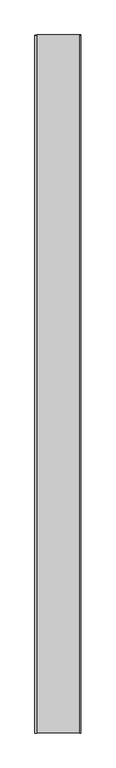
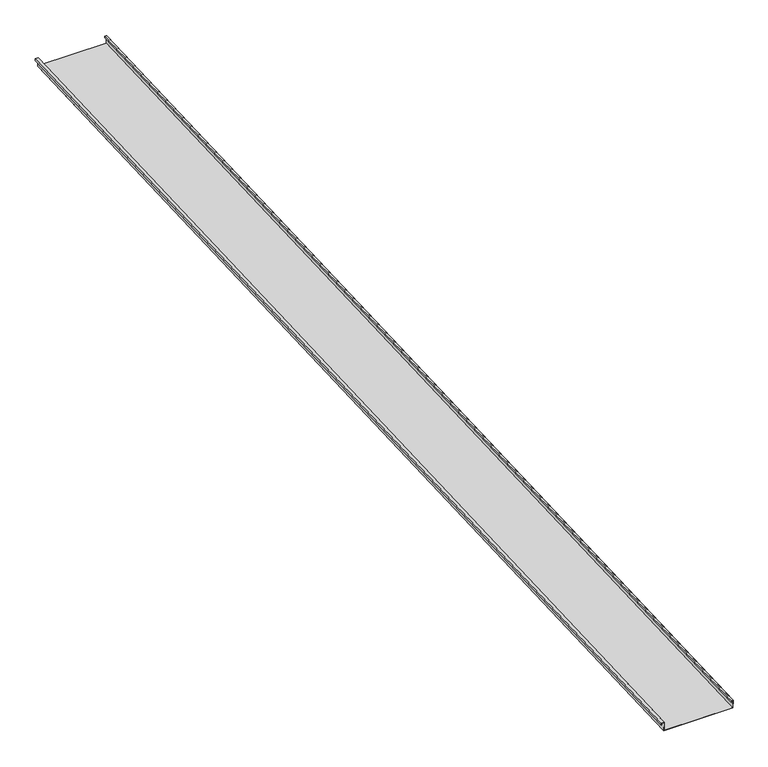
"""IFC4 building model written with IfcOpenShell, lengths in millimetres: proxy geometry, Generic Models 2:Generic Models 2:310765:Generic Models 2:310765 : Generic Models 2:Generic Models 2:310765:125 : Generic Models 2:Generic Models 2:310765:Generic Models 2:310765 : Generic Models 2:Generic Models 2:310765:300385."""

from ifc_helpers import new_model, si_unit, frame, origin, place, context, project, spatial, polyline, outline, extrude, source, transform, mapped, element, save


def generic_models_6f656777(model_context):
    return source(origin(), model_context, "Body", "SweptSolid", [
        extrude(outline(polyline([(1.5875, 0.0), (1.5875, 50.8), (407.9875, 50.8), (407.9875, 1.5875), (396.875, 1.5875), (396.875, 11.1125), (398.4625, 11.1125), (398.4625, 3.175), (406.4, 3.175), (406.4, 49.2125), (3.175, 49.2125), (3.175, -1.5874999), (-14.2875, -1.5874999), (-14.2875, 9.525), (-12.7, 9.525), (-12.7, 0.0), (1.5875, 0.0)])), frame((663392.5596405, -581354.4345603, 3902.6697972), z_axis=(0.0, 0.9991330730923568, 0.041630544712067834), x_axis=(1.0, 0.0, 0.0)), (0.0, 0.0, 1.0), 6400.8),
    ])


if __name__ == "__main__":
    model = new_model("IFC4")
    model_context = context("Model", 3, world=origin())
    ifc_project = project(units=[si_unit("LENGTHUNIT", "METRE", prefix="MILLI")], contexts=[model_context])
    site = spatial("IfcSite", under=ifc_project)
    building = spatial("IfcBuilding", under=site)
    placement = place(None, origin())
    generic_models_shape = generic_models_6f656777(model_context)
    element("IfcBuildingElementProxy", 1, Name="Generic Models 2:Generic Models 2:310765:Generic Models 2:310765 : Generic Models 2:Generic Models 2:310765:125 : Generic Models 2:Generic Models 2:310765:Generic Models 2:310765 : Generic Models 2:Generic Models 2:310765:300385", ObjectType="Generic Models 2:Generic Models 2:310765:Generic Models 2:310765 : Generic Models 2:Generic Models 2:310765:125 : Generic Models 2:Generic Models 2:310765:Generic Models 2:310765 : Generic Models 2:Generic Models 2:310765:300385", at=placement, inside=building, context=model_context, shape_type="MappedRepresentation", body=[
        mapped(generic_models_shape, transform((0.0, 0.0, 0.0), x_axis=(1.0, 0.0, 0.0), y_axis=(0.0, 1.0, 0.0), z_axis=(0.0, 0.0, 1.0))),
    ])
    save(model, "model.ifc")

# Revit data of these elements
# Type "Generic Models 2:Generic Models 2:310765:Generic Models 2:310765 : Generic Models 2:Generic Models 2:310765:125 : Generic Models 2:Generic Models 2:310765:Generic Models 2:310765 : Generic Models 2:Generic Models 2:310765:300385"
#   NameOverride = "Generic Models 2:Generic Models 2:310765:Generic Models 2:310765 : Generic Models 2:Generic Models 2:310765:300385"
#   ObjectTypeOverride = "Generic Models 2:310765 : Generic Models 2:Generic Models 2:310765"
#   Reference = "Generic Models 2"
#   Tag = "300385"
# Element 1 (IfcBuildingElementProxy, "Generic Models 2:Generic Models 2:310765:Generic Models 2:310765 : Generic Models 2:Generic Models 2:310765:125 : Generic Models 2:Generic Models 2:310765:Generic Models 2:310765 : Generic Models 2:Generic Models 2:310765:300385")
#   Materials on its faces: "THERMAL BROKEN ALUMINUM STOREFRONT FOR POLYCARBONATE"
# Materials
#   "THERMAL BROKEN ALUMINUM STOREFRONT FOR POLYCARBONATE": class "Unassigned", colour RGB 244 244 244, transparency 0, Keynote = "M07611300.01", Cost = 0
